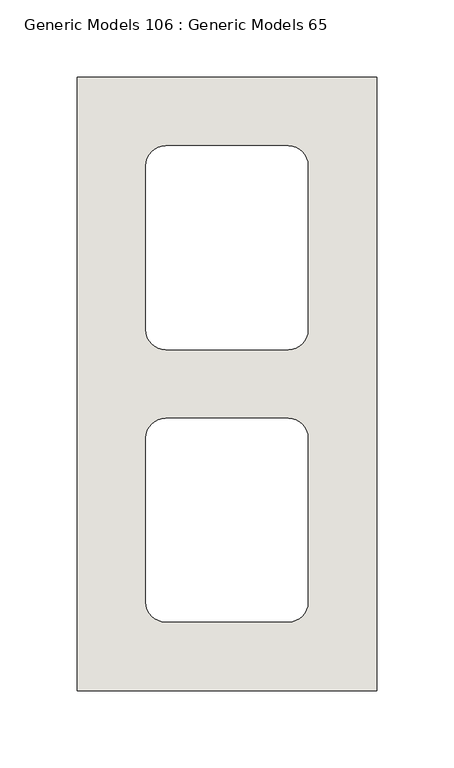
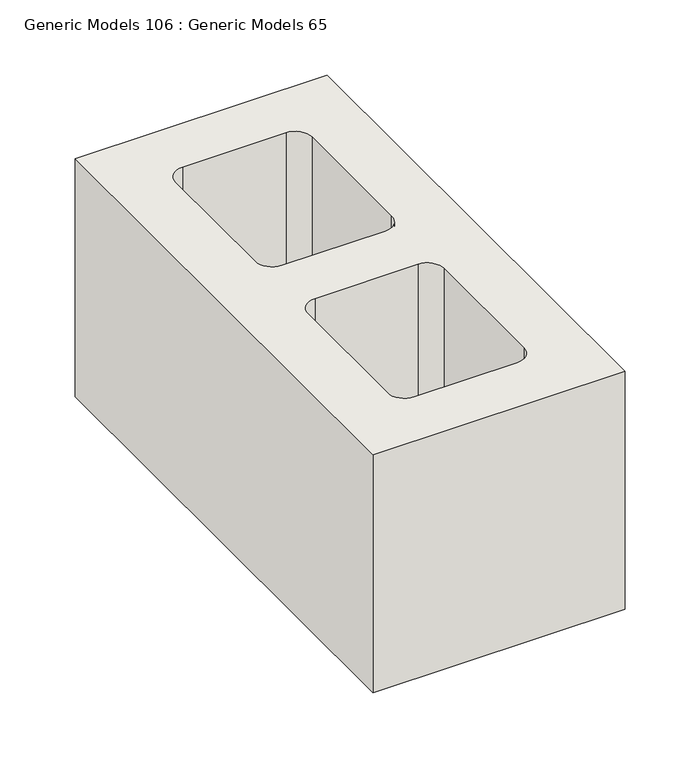
"""IFC4 building model written with IfcOpenShell, lengths in millimetres: wall geometry, Generic Models 106 : Generic Models 65."""

from ifc_helpers import new_model, si_unit, point, frame, frame_2d, origin, place, context, project, spatial, polyline, circle_curve, trimmed, segment, composite_curve, outline, extrude, source, transform, mapped, element, save


def generic_models_106_generic_models_65_06748fca(model_context):
    return source(origin(), model_context, "Body", "SweptSolid", [
        extrude(outline(polyline([(375486.6125, 292.1), (375292.9375, 292.1), (375292.9375, 688.975), (375486.6125, 688.975), (375486.6125, 292.1)]), holes=[composite_curve([segment(polyline([(375442.1625, 525.4625), (375442.1625, 631.825)]), True, "CONTINUOUS"), segment(trimmed(circle_curve(frame_2d((375429.4625, 631.825)), 12.7), [point((375442.1625, 631.825))], [point((375429.4625, 644.525))], True, "CARTESIAN"), True, "CONTINUOUS"), segment(polyline([(375429.4625, 644.525), (375350.0875, 644.525)]), True, "CONTINUOUS"), segment(trimmed(circle_curve(frame_2d((375350.0875, 631.825)), 12.7), [point((375350.0875, 644.525))], [point((375337.3875, 631.825))], True, "CARTESIAN"), True, "CONTINUOUS"), segment(polyline([(375337.3875, 631.825), (375337.3875, 525.4625)]), True, "CONTINUOUS"), segment(trimmed(circle_curve(frame_2d((375350.0875, 525.4625)), 12.7), [point((375337.3875, 525.4625))], [point((375350.0875, 512.7625))], True, "CARTESIAN"), True, "CONTINUOUS"), segment(polyline([(375350.0875, 512.7625), (375429.4625, 512.7625)]), True, "CONTINUOUS"), segment(trimmed(circle_curve(frame_2d((375429.4625, 525.4625)), 12.7), [point((375429.4625, 512.7625))], [point((375442.1625, 525.4625))], True, "CARTESIAN"), True, "CONTINUOUS")], self_intersect=False), composite_curve([segment(polyline([(375337.3875, 455.6125), (375337.3875, 349.25)]), True, "CONTINUOUS"), segment(trimmed(circle_curve(frame_2d((375350.0875, 349.25)), 12.7), [point((375337.3875, 349.25))], [point((375350.0875, 336.55))], True, "CARTESIAN"), True, "CONTINUOUS"), segment(polyline([(375350.0875, 336.55), (375429.4625, 336.55)]), True, "CONTINUOUS"), segment(trimmed(circle_curve(frame_2d((375429.4625, 349.25)), 12.7), [point((375429.4625, 336.55))], [point((375442.1625, 349.25))], True, "CARTESIAN"), True, "CONTINUOUS"), segment(polyline([(375442.1625, 349.25), (375442.1625, 455.6125)]), True, "CONTINUOUS"), segment(trimmed(circle_curve(frame_2d((375429.4625, 455.6125)), 12.7), [point((375442.1625, 455.6125))], [point((375429.4625, 468.3125))], True, "CARTESIAN"), True, "CONTINUOUS"), segment(polyline([(375429.4625, 468.3125), (375350.0875, 468.3125)]), True, "CONTINUOUS"), segment(trimmed(circle_curve(frame_2d((375350.0875, 455.6125)), 12.7), [point((375350.0875, 468.3125))], [point((375337.3875, 455.6125))], True, "CARTESIAN"), True, "CONTINUOUS")], self_intersect=False)]), frame((0.0, 0.0, 2549.525), z_axis=(0.0, 0.0, 1.0), x_axis=(1.0, 0.0, 0.0)), (0.0, 0.0, 1.0), 193.675),
    ])


if __name__ == "__main__":
    model = new_model("IFC4")
    model_context = context("Model", 3, world=origin())
    ifc_project = project(units=[si_unit("LENGTHUNIT", "METRE", prefix="MILLI")], contexts=[model_context])
    site = spatial("IfcSite", under=ifc_project)
    building = spatial("IfcBuilding", under=site)
    placement = place(None, origin())
    generic_models_106_generic_models_65_shape = generic_models_106_generic_models_65_06748fca(model_context)
    element("IfcWall", 1, ObjectType="Generic Models 106 : Generic Models 65", at=placement, inside=building, context=model_context, shape_type="MappedRepresentation", body=[
        mapped(generic_models_106_generic_models_65_shape, transform((0.0, 0.0, 0.0), x_axis=(1.0, 0.0, 0.0), y_axis=(0.0, 1.0, 0.0), z_axis=(0.0, 0.0, 1.0))),
    ])
    save(model, "model.ifc")

# Revit data of these elements
# Element 1 (IfcWall, "Generic Models 106 : Generic Models 65")
#   Materials on its faces: "CMU (SEE 'WALL TAG' FOR SIZE)"
# Materials
#   "CMU (SEE 'WALL TAG' FOR SIZE)": class "Masonry", colour RGB 203 203 199, transparency 0, Description = "Concrete masonry units", Cost = 0
